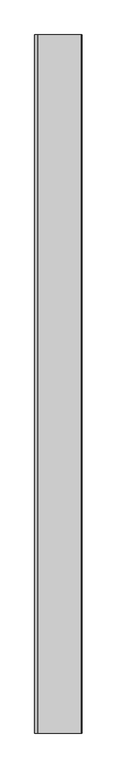
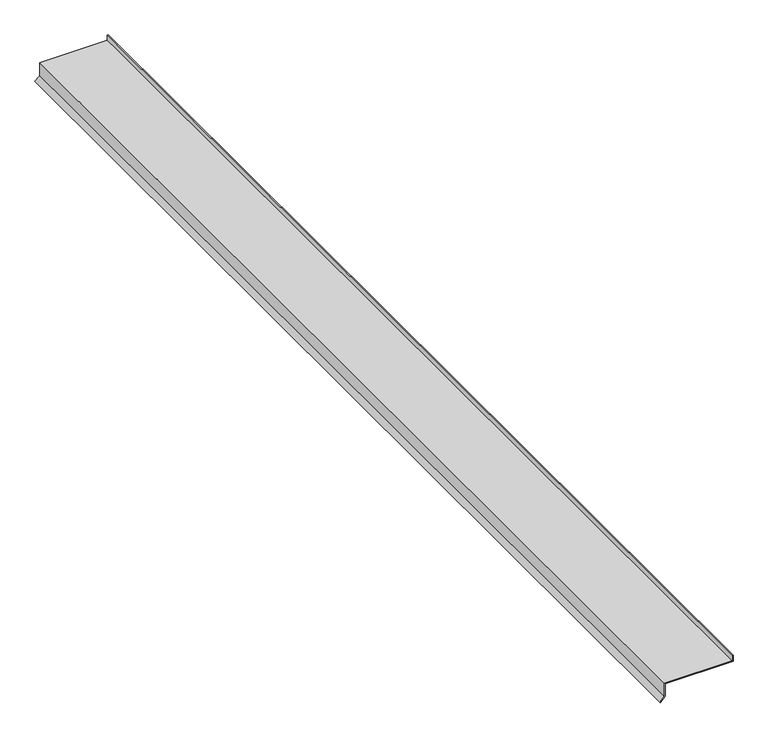
"""IFC4 building model written with IfcOpenShell, lengths in millimetres: proxy geometry, Flashing027 4116 : Flashing027 4116."""

from ifc_helpers import new_model, si_unit, frame, origin, place, context, project, spatial, polyline, outline, extrude, source, transform, mapped, element, save


def generic_models_c57af108(model_context):
    return source(origin(), model_context, "Body", "SweptSolid", [
        extrude(outline(polyline([(40335.3398438, -986.5449829), (40325.640625, -986.5449829), (40325.640625, -1111.5771484), (40300.3872772, -1111.5771484), (40291.9157249, -1120.4555041), (40290.46875, -1119.0748291), (40299.53125, -1109.5771484), (40323.640625, -1109.5771484), (40323.640625, -984.5449829), (40335.3398438, -984.5449829), (40335.3398438, -986.5449829)])), frame((0.0, -1052.8906574, 0.0), z_axis=(0.0, 1.0, 0.0), x_axis=(0.0, 0.0, 1.0)), (0.0, 0.0, 1.0), 2000.0),
    ])


if __name__ == "__main__":
    model = new_model("IFC4")
    model_context = context("Model", 3, world=origin())
    ifc_project = project(units=[si_unit("LENGTHUNIT", "METRE", prefix="MILLI")], contexts=[model_context])
    site = spatial("IfcSite", under=ifc_project)
    building = spatial("IfcBuilding", under=site)
    placement = place(None, origin())
    generic_models_shape = generic_models_c57af108(model_context)
    element("IfcBuildingElementProxy", 1, Name="Flashing027 4116 : Flashing027 4116", ObjectType="Flashing027 4116 : Flashing027 4116", at=placement, inside=building, context=model_context, shape_type="MappedRepresentation", body=[
        mapped(generic_models_shape, transform((0.0, 0.0, 0.0), x_axis=(1.0, 0.0, 0.0), y_axis=(0.0, 1.0, 0.0), z_axis=(0.0, 0.0, 1.0))),
    ])
    save(model, "model.ifc")

# Revit data of these elements
# Type "Flashing027 4116 : Flashing027 4116"
#   NameOverride = "Flashing027"
# Element 1 (IfcBuildingElementProxy, "Flashing027 4116 : Flashing027 4116")
#   Materials on its faces: "SILL PAN"
# Materials
#   "SILL PAN": class "Unassigned", colour RGB 255 170 255, transparency 0
